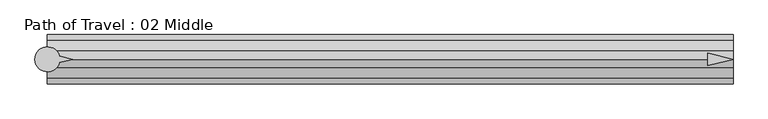
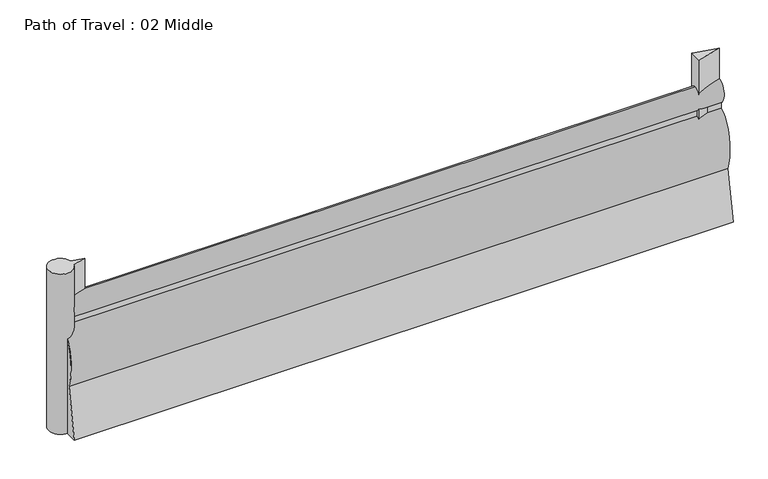
"""IFC4 building model written with IfcOpenShell, lengths in millimetres: proxy geometry, Path of Travel : 02 Middle."""

import ifcopenshell
import ifcopenshell.guid

model = None  # the IFC model being written
_history = None  # IfcOwnerHistory: only IFC2X3 demands one
_inside = {}  # id of a spatial element -> (the spatial element, [elements in it])
_under = {}  # id of a project, library or spatial element -> (it, [spatial elements below it])
_declared = {}  # id of a project -> (the project, [libraries it declares])
_typed = {}  # id of a type object -> (the type object, [elements of that type])
_made_of = {}  # id of a material, layer set ... -> (it, [elements and type objects made of it])


def new_model(schema):
    """Start an empty IFC model of exactly this schema.

    Asked for "IFC4X3", IfcOpenShell would pick the latest addendum, in which some entities
    have other attributes; the version numbers below select the first issue.
    IFC2X3 requires an IfcOwnerHistory on every rooted entity: one is made here for all.
    """
    global model, _history
    if schema == "IFC4X3":
        model = ifcopenshell.file(schema_version=(4, 3, 0, 0))
    else:
        model = ifcopenshell.file(schema=schema)
    _inside.clear()
    _under.clear()
    _declared.clear()
    _typed.clear()
    _made_of.clear()
    _history = None
    if model.schema == "IFC2X3":
        org = make("IfcOrganization", Name="unknown")
        user = make(
            "IfcPersonAndOrganization",
            ThePerson=make("IfcPerson", FamilyName="unknown"),
            TheOrganization=org,
        )
        app = make(
            "IfcApplication",
            ApplicationDeveloper=org,
            Version="unknown",
            ApplicationFullName="unknown",
            ApplicationIdentifier="unknown",
        )
        _history = make(
            "IfcOwnerHistory",
            OwningUser=user,
            OwningApplication=app,
            ChangeAction="ADDED",
            CreationDate=0,
        )
    return model


def make(cls, **values):
    """One entity of the class cls with the attributes given. An attribute that is None is left unset."""
    return model.create_entity(
        cls, **{name: value for name, value in values.items() if value is not None}
    )


def rooted(cls, **values):
    """An entity with a GlobalId (a new one), such as an element, a storey or a relation."""
    return make(cls, GlobalId=ifcopenshell.guid.new(), OwnerHistory=_history, **values)


def si_unit(unit_type, name, prefix=None):
    """IfcSIUnit, for example si_unit("LENGTHUNIT", "METRE", prefix="MILLI")."""
    return make("IfcSIUnit", UnitType=unit_type, Prefix=prefix, Name=name)


def assignment(units):
    """IfcUnitAssignment: the units of a project."""
    return None if units is None else make("IfcUnitAssignment", Units=units)


def point(xyz):
    """IfcCartesianPoint."""
    return None if xyz is None else make("IfcCartesianPoint", Coordinates=xyz)


def direction(xyz):
    """IfcDirection."""
    return None if xyz is None else make("IfcDirection", DirectionRatios=xyz)


def frame(location, z_axis=None, x_axis=None):
    """IfcAxis2Placement3D, a coordinate frame: its origin and axes. An axis left out is left unset."""
    return make(
        "IfcAxis2Placement3D",
        Location=point(location),
        Axis=direction(z_axis),
        RefDirection=direction(x_axis),
    )


def frame_2d(location, x_axis=None):
    """IfcAxis2Placement2D, a coordinate frame in the plane: its origin and x axis."""
    return make(
        "IfcAxis2Placement2D", Location=point(location), RefDirection=direction(x_axis)
    )


def origin():
    """The frame at (0, 0, 0) with its axes left unset."""
    return frame((0.0, 0.0, 0.0))


def origin_with_axes():
    """The frame at (0, 0, 0) with the z axis (0, 0, 1) and the x axis (1, 0, 0) written out."""
    return frame((0.0, 0.0, 0.0), z_axis=(0.0, 0.0, 1.0), x_axis=(1.0, 0.0, 0.0))


def place(relative_to, where):
    """IfcLocalPlacement: puts the frame where relative to a parent placement (None: the world)."""
    return make(
        "IfcLocalPlacement", PlacementRelTo=relative_to, RelativePlacement=where
    )


def context(
    kind, dimensions, precision=None, world=None, true_north=None, identifier=None
):
    """IfcGeometricRepresentationContext, for example the 3D "Model" context."""
    return make(
        "IfcGeometricRepresentationContext",
        ContextIdentifier=identifier,
        ContextType=kind,
        CoordinateSpaceDimension=dimensions,
        Precision=precision,
        WorldCoordinateSystem=world,
        TrueNorth=true_north,
    )


def project(units=None, contexts=None):
    """IfcProject with its units and contexts."""
    return rooted(
        "IfcProject",
        Name="project",
        RepresentationContexts=contexts,
        UnitsInContext=assignment(units),
    )


def spatial(cls, under=None, at=None, **own):
    """A site, building, storey or space (cls), placed at a placement, below another one or the project."""
    s = rooted(cls, ObjectPlacement=at, **own)
    if under is not None:
        _under.setdefault(under.id(), (under, []))[1].append(s)
    return s


def polyline(points):
    """IfcPolyline through the points."""
    return make("IfcPolyline", Points=[point(p) for p in points])


def circle_curve(where, radius):
    """IfcCircle in the frame where."""
    return make("IfcCircle", Position=where, Radius=radius)


def ellipse_curve(where, semi_axis1, semi_axis2):
    """IfcEllipse in the frame where."""
    return make(
        "IfcEllipse", Position=where, SemiAxis1=semi_axis1, SemiAxis2=semi_axis2
    )


def trimmed(basis, trim1, trim2, sense, master):
    """IfcTrimmedCurve: the piece of a basis curve between two trims."""
    return make(
        "IfcTrimmedCurve",
        BasisCurve=basis,
        Trim1=trim1,
        Trim2=trim2,
        SenseAgreement=sense,
        MasterRepresentation=master,
    )


def segment(curve, same_sense, transition):
    """IfcCompositeCurveSegment."""
    return make(
        "IfcCompositeCurveSegment",
        Transition=transition,
        SameSense=same_sense,
        ParentCurve=curve,
    )


def composite_curve(segments, self_intersect=None):
    """IfcCompositeCurve: segments joined end to end."""
    return make("IfcCompositeCurve", Segments=segments, SelfIntersect=self_intersect)


def outline(outer, holes=None, kind="AREA"):
    """IfcArbitraryClosedProfileDef: a profile drawn as a closed curve; with holes, ...WithVoids."""
    if holes is None:
        return make("IfcArbitraryClosedProfileDef", ProfileType=kind, OuterCurve=outer)
    return make(
        "IfcArbitraryProfileDefWithVoids",
        ProfileType=kind,
        OuterCurve=outer,
        InnerCurves=holes,
    )


def extrude(swept, where, along, depth):
    """IfcExtrudedAreaSolid: the profile swept, set in the frame where, extruded along a direction by depth."""
    return make(
        "IfcExtrudedAreaSolid",
        SweptArea=swept,
        Position=where,
        ExtrudedDirection=direction(along),
        Depth=depth,
    )


def shape(context_of_items, identifier, shape_type, items):
    """IfcShapeRepresentation: the items that make up one representation, for example the "Body"."""
    return make(
        "IfcShapeRepresentation",
        ContextOfItems=context_of_items,
        RepresentationIdentifier=identifier,
        RepresentationType=shape_type,
        Items=items,
    )


def source(mapping_origin, context_of_items, identifier, shape_type, items):
    """IfcRepresentationMap: a shape defined once, which mapped items show again and again."""
    return make(
        "IfcRepresentationMap",
        MappingOrigin=mapping_origin,
        MappedRepresentation=shape(context_of_items, identifier, shape_type, items),
    )


def transform(
    local_origin,
    x_axis=None,
    y_axis=None,
    z_axis=None,
    scale=None,
    scale2=None,
    scale3=None,
    uniform=True,
):
    """IfcCartesianTransformationOperator3D, or its non-uniform kind. x_axis, y_axis, z_axis: its Axis1, 2, 3."""
    if uniform:
        return make(
            "IfcCartesianTransformationOperator3D",
            Axis1=direction(x_axis),
            Axis2=direction(y_axis),
            LocalOrigin=point(local_origin),
            Scale=scale,
            Axis3=direction(z_axis),
        )
    return make(
        "IfcCartesianTransformationOperator3DnonUniform",
        Axis1=direction(x_axis),
        Axis2=direction(y_axis),
        LocalOrigin=point(local_origin),
        Scale=scale,
        Axis3=direction(z_axis),
        Scale2=scale2,
        Scale3=scale3,
    )


def mapped(mapping_source, mapping_target):
    """IfcMappedItem: shows the shape of a source again, moved by a transform."""
    return make(
        "IfcMappedItem", MappingSource=mapping_source, MappingTarget=mapping_target
    )


def made_of(thing, what):
    """Note that an element or type object is made of a material, layer set ...; save() writes the relation."""
    if what is not None:
        _made_of.setdefault(what.id(), (what, []))[1].append(thing)
    return thing


def element(
    cls,
    number,
    at=None,
    inside=None,
    cuts=None,
    type_object=None,
    material=None,
    context=None,
    identifier="Body",
    shape_type=None,
    held_by="IfcProductDefinitionShape",
    body=None,
    shapes=None,
    **own,
):
    """One element of the class cls, such as IfcWall. Its Tag is "e" and its number.

    at: its placement. inside: the storey or other place that contains it. cuts: it is an
    opening in that element (IfcRelVoidsElement). A single representation is given by context,
    identifier, shape_type and body (its items); several are given by shapes. held_by: the class
    of the entity that holds the representations. save() writes the other relations.
    """
    e = rooted(cls, Tag="e%d" % number, ObjectPlacement=at, **own)
    if body is not None:
        shapes = [shape(context, identifier, shape_type, body)]
    if shapes is not None:
        e.Representation = make(held_by, Representations=shapes)
    if inside is not None:
        _inside.setdefault(inside.id(), (inside, []))[1].append(e)
    if cuts is not None:
        rooted(
            "IfcRelVoidsElement", RelatingBuildingElement=cuts, RelatedOpeningElement=e
        )
    if type_object is not None:
        _typed.setdefault(type_object.id(), (type_object, []))[1].append(e)
    return made_of(e, material)


def aggregate(whole, parts):
    """IfcRelAggregates: a whole, such as a stair, and the parts it consists of."""
    return rooted("IfcRelAggregates", RelatingObject=whole, RelatedObjects=parts)


def save(model, path):
    """Write the relations noted so far, then the file.

    IfcRelAggregates (storeys below a building ...), IfcRelContainedInSpatialStructure (elements
    in a storey), IfcRelDefinesByType, IfcRelAssociatesMaterial and IfcRelDeclares: one each for
    every whole, place, type object, material and project.
    """
    for whole, parts in _under.values():
        aggregate(whole, parts)
    for where, things in _inside.values():
        rooted(
            "IfcRelContainedInSpatialStructure",
            RelatedElements=things,
            RelatingStructure=where,
        )
    for kind, things in _typed.values():
        rooted("IfcRelDefinesByType", RelatedObjects=things, RelatingType=kind)
    for what, things in _made_of.values():
        rooted("IfcRelAssociatesMaterial", RelatedObjects=things, RelatingMaterial=what)
    for by, libraries in _declared.values():
        rooted("IfcRelDeclares", RelatingContext=by, RelatedDefinitions=libraries)
    model.write(path)


def plane_surface(at):
    """IfcPlane: the flat surface through the origin of the frame at, square to its z axis."""
    return make("IfcPlane", Position=at)


def extruded_surface(curve, direction_of_extrusion, depth):
    """IfcSurfaceOfLinearExtrusion: the curve pushed along a direction by depth."""
    return make(
        "IfcSurfaceOfLinearExtrusion",
        SweptCurve=make("IfcArbitraryOpenProfileDef", ProfileType="CURVE", Curve=curve),
        ExtrudedDirection=direction(direction_of_extrusion),
        Depth=depth,
    )


def advanced_brep(points, edges, surfaces, faces):
    """IfcAdvancedBrep: a solid bounded by faces that lie on surfaces and meet in shared edges.

    An edge is (start, end): straight between two places in points (the first is 0);
    or (start, end, curve); or (start, end, curve, False) where it runs against its curve.
    A face is (place in surfaces, loops), or (place, loops, False) where it looks against
    its surface's normal. A loop lists edges by number (the first is 1), with a minus sign
    where the edge is run from its end to its start. The first loop is the outer one.
    """
    corners = [point(p) for p in points]
    vertices = [make("IfcVertexPoint", VertexGeometry=c) for c in corners]
    made = []
    for start, end, *more in edges:
        made.append(
            make(
                "IfcEdgeCurve",
                EdgeStart=vertices[start],
                EdgeEnd=vertices[end],
                EdgeGeometry=more[0] if more else make("IfcPolyline", Points=[corners[start], corners[end]]),
                SameSense=more[1] if len(more) > 1 else True,
            )
        )
    hull = []
    for where, loops, *sense in faces:
        bounds = []
        for j, loop in enumerate(loops):
            ring = [make("IfcOrientedEdge", EdgeElement=made[abs(k) - 1], Orientation=k > 0) for k in loop]
            bounds.append(
                make(
                    "IfcFaceOuterBound" if j == 0 else "IfcFaceBound",
                    Bound=make("IfcEdgeLoop", EdgeList=ring),
                    Orientation=True,
                )
            )
        hull.append(make("IfcAdvancedFace", Bounds=bounds, FaceSurface=surfaces[where], SameSense=sense[0] if sense else True))
    return make("IfcAdvancedBrep", Outer=make("IfcClosedShell", CfsFaces=hull))


def path_of_travel_02_middle_f1e6894a(model_context):
    return source(origin(), model_context, "Body", "SolidModel", [
        advanced_brep(
        [(227.5554837, 0.0, 1727.2), (227.5554837, 42.9018657, 1436.6534209), (227.5554837, 42.9018657, 1363.4763406), (227.5554837, 184.1186263, 643.4144547), (227.5554837, 297.5699544, 0.0), (227.5554837, 145.6574193, 0.0), (227.5554837, 0.0, 584.2), (227.5554837, -145.6574193, 0.0), (227.5554837, -297.5699544, 0.0), (227.5554837, -184.1186263, 643.4144547), (227.5554837, -42.9018657, 1363.4763406), (227.5554837, -42.9018657, 1436.6534209), (8507.3212956, 0.0, 1727.2), (8507.3212956, -42.9018657, 1436.6534209), (8507.3212956, -42.9018657, 1363.4763406), (8507.3212956, -184.1186263, 643.4144547), (8507.3212956, -297.5699544, 0.0), (8507.3212956, -145.6574193, 0.0), (8507.3212956, 0.0, 584.2), (8507.3212956, 145.6574193, 0.0), (8507.3212956, 297.5699544, 0.0), (8507.3212956, 184.1186263, 643.4144547), (8507.3212956, 42.9018657, 1363.4763406), (8507.3212956, 42.9018657, 1436.6534209)],
        [
            (0, 1, ellipse_curve(frame((227.5554837, 0.0, 1574.8), z_axis=(-1.0, 0.0, 0.0), x_axis=(0.0, 0.0, 1.0)), 152.4, 101.6)),
            (1, 2),
            (2, 3, ellipse_curve(frame((227.5554837, 0.0, 914.4), z_axis=(-1.0, 0.0, 0.0), x_axis=(0.0, 0.0, -1.0)), 457.2, 228.6)),
            (3, 4),
            (4, 5),
            (5, 6),
            (6, 7),
            (7, 8),
            (8, 9),
            (9, 10, ellipse_curve(frame((227.5554837, 0.0, 914.4), z_axis=(-1.0, 0.0, 0.0), x_axis=(0.0, 0.0, -1.0)), 457.2, 228.6)),
            (10, 11),
            (11, 0, ellipse_curve(frame((227.5554837, 0.0, 1574.8), z_axis=(-1.0, 0.0, 0.0), x_axis=(0.0, 0.0, 1.0)), 152.4, 101.6)),
            (12, 13, ellipse_curve(frame((8507.3212956, 0.0, 1574.8), z_axis=(1.0, 0.0, 0.0), x_axis=(0.0, 0.0, 1.0)), 152.4, 101.6)),
            (13, 14),
            (14, 15, ellipse_curve(frame((8507.3212956, 0.0, 914.4), z_axis=(1.0, 0.0, 0.0), x_axis=(0.0, 0.0, -1.0)), 457.2, 228.6)),
            (15, 16),
            (16, 17),
            (17, 18),
            (18, 19),
            (19, 20),
            (20, 21),
            (21, 22, ellipse_curve(frame((8507.3212956, 0.0, 914.4), z_axis=(1.0, 0.0, 0.0), x_axis=(0.0, 0.0, -1.0)), 457.2, 228.6)),
            (22, 23),
            (23, 12, ellipse_curve(frame((8507.3212956, 0.0, 1574.8), z_axis=(1.0, 0.0, 0.0), x_axis=(0.0, 0.0, 1.0)), 152.4, 101.6)),
            (0, 12),
            (23, 1),
            (22, 2),
            (21, 3),
            (20, 4),
            (19, 5),
            (18, 6),
            (17, 7),
            (16, 8),
            (15, 9),
            (14, 10),
            (13, 11),
        ],
        [
            plane_surface(frame((227.5554837, 0.0, 0.0), z_axis=(-1.0, 0.0, 0.0), x_axis=(0.0, 0.0, 1.0))),
            plane_surface(frame((8507.3212956, 0.0, 0.0), z_axis=(1.0, 0.0, 0.0), x_axis=(0.0, 0.0, 1.0))),
            extruded_surface(trimmed(ellipse_curve(frame((8507.3212956, 0.0, 1574.8), z_axis=(-1.0, 0.0, 0.0), x_axis=(0.0, 0.0, 1.0)), 152.4, 101.6), [point((8507.3212956, 0.0, 1727.2))], [point((8507.3212956, 42.9018657, 1436.6534209))], True, "CARTESIAN"), (-8279.7658119, 0.0, 0.0), 8279.7658119),
            plane_surface(frame((227.5554837, 42.9018657, 1436.6534209), z_axis=(0.0, 1.0, 0.0), x_axis=(1.0, 0.0, 0.0))),
            extruded_surface(trimmed(ellipse_curve(frame((8507.3212956, 0.0, 914.4), z_axis=(-1.0, 0.0, 0.0), x_axis=(0.0, 0.0, -1.0)), 457.2, 228.6), [point((8507.3212956, 42.9018657, 1363.4763406))], [point((8507.3212956, 184.1186263, 643.4144547))], True, "CARTESIAN"), (-8279.7658119, 0.0, 0.0), 8279.7658119),
            plane_surface(frame((227.5554837, 184.1186263, 643.4144547), z_axis=(0.0, 0.9848077530122078, 0.1736481776669322), x_axis=(1.0, 0.0, 0.0))),
            plane_surface(frame((227.5554837, 297.5699544, 0.0), z_axis=(0.0, 0.0, -1.0), x_axis=(1.0, 0.0, 0.0))),
            plane_surface(frame((227.5554837, 145.6574193, 0.0), z_axis=(0.0, -0.9702957262760199, -0.2419218955995739), x_axis=(1.0, 0.0, 0.0))),
            plane_surface(frame((227.5554837, 0.0, 584.2), z_axis=(0.0, 0.9702957262759961, -0.24192189559966923), x_axis=(1.0, 0.0, 0.0))),
            plane_surface(frame((227.5554837, -145.6574193, 0.0), z_axis=(0.0, 0.0, -1.0), x_axis=(1.0, 0.0, 0.0))),
            plane_surface(frame((227.5554837, -297.5699544, 0.0), z_axis=(0.0, -0.984807753012208, 0.17364817766693066), x_axis=(1.0, 0.0, 0.0))),
            extruded_surface(trimmed(ellipse_curve(frame((8507.3212956, 0.0, 914.4), z_axis=(-1.0, 0.0, 0.0), x_axis=(0.0, 0.0, -1.0)), 457.2, 228.6), [point((8507.3212956, -184.1186263, 643.4144547))], [point((8507.3212956, -42.9018657, 1363.4763406))], True, "CARTESIAN"), (-8279.7658119, 0.0, 0.0), 8279.7658119),
            plane_surface(frame((227.5554837, -42.9018657, 1363.4763406), z_axis=(0.0, -1.0, 0.0), x_axis=(1.0, 0.0, 0.0))),
            extruded_surface(trimmed(ellipse_curve(frame((8507.3212956, 0.0, 1574.8), z_axis=(-1.0, 0.0, 0.0), x_axis=(0.0, 0.0, 1.0)), 152.4, 101.6), [point((8507.3212956, -42.9018657, 1436.6534209))], [point((8507.3212956, 0.0, 1727.2))], True, "CARTESIAN"), (-8279.7658119, 0.0, 0.0), 8279.7658119),
        ],
        [
            (0, [[1, 2, 3, 4, 5, 6, 7, 8, 9, 10, 11, 12]]),
            (1, [[13, 14, 15, 16, 17, 18, 19, 20, 21, 22, 23, 24]]),
            (2, [[-1, 25, -24, 26]]),
            (3, [[-2, -26, -23, 27]]),
            (4, [[-3, -27, -22, 28]]),
            (5, [[-4, -28, -21, 29]]),
            (6, [[-5, -29, -20, 30]]),
            (7, [[-6, -30, -19, 31]]),
            (8, [[-7, -31, -18, 32]]),
            (9, [[-8, -32, -17, 33]]),
            (10, [[-9, -33, -16, 34]]),
            (11, [[-10, -34, -15, 35]]),
            (12, [[-11, -35, -14, 36]]),
            (13, [[-12, -36, -13, -25]]),
        ],
    ),
        extrude(outline(polyline([(8201.316149, 76.2006338), (8507.3212956, 0.0), (8201.316149, -76.2006338), (8201.316149, 76.2006338)])), origin_with_axes(), (0.0, 0.0, 1.0), 2129.5973753),
        extrude(outline(composite_curve([segment(polyline([(372.7837828, 39.4440225), (531.182385, 0.0), (372.7837828, -39.4440225)]), True, "CONTINUOUS"), segment(trimmed(circle_curve(frame_2d((227.2200886, 0.0)), 150.8131956), [point((372.7837828, -39.4440225))], [point((372.7837828, 39.4440225))], False, "CARTESIAN"), True, "CONTINUOUS")], self_intersect=False)), origin_with_axes(), (0.0, 0.0, 1.0), 2129.5973753),
    ])


if __name__ == "__main__":
    model = new_model("IFC4")
    model_context = context("Model", 3, world=origin())
    ifc_project = project(units=[si_unit("LENGTHUNIT", "METRE", prefix="MILLI")], contexts=[model_context])
    site = spatial("IfcSite", under=ifc_project)
    building = spatial("IfcBuilding", under=site)
    placement = place(None, origin())
    path_of_travel_02_middle_shape = path_of_travel_02_middle_f1e6894a(model_context)
    element("IfcBuildingElementProxy", 1, Name="Path of Travel : 02 Middle", ObjectType="Path of Travel : 02 Middle", at=placement, inside=building, context=model_context, shape_type="MappedRepresentation", body=[
        mapped(path_of_travel_02_middle_shape, transform((0.0, 0.0, 0.0), x_axis=(1.0, 0.0, 0.0), y_axis=(0.0, 1.0, 0.0), z_axis=(0.0, 0.0, 1.0))),
    ])
    save(model, "model.ifc")

# Revit data of these elements
# Type "Path of Travel : 02 Middle"
#   Path of Egress [instance default] = 4' - 0"
#   built-in parameter 1001306 [instance default] = 4 (stored number, unit not read)
#   Dot at Start = no
#   Arrow in Middle = yes
#   Arrow at End = no
#   Egress Path = none
# Element 1 (IfcBuildingElementProxy, "Path of Travel : 02 Middle")
#   Path of Egress = 27' - 1.97503"
#   built-in parameter 1001306 = 27.1646 (stored number, unit not read)
